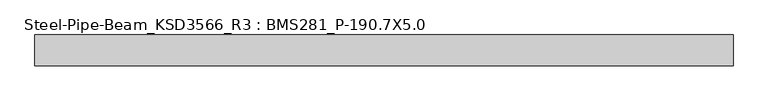
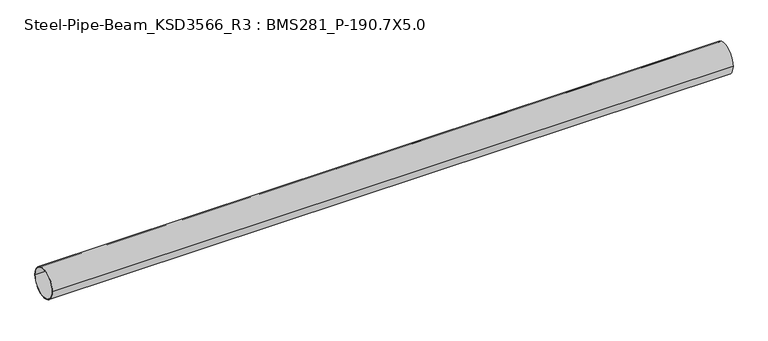
"""IFC4 building model written with IfcOpenShell, lengths in millimetres: member geometry, Steel-Pipe-Beam_KSD3566_R3 : BMS281_P-190.7X5.0."""

from ifc_helpers import new_model, si_unit, point, frame, origin, origin_2d, place, context, project, spatial, circle_curve, trimmed, segment, composite_curve, outline, extrude, source, transform, mapped, element, save


def steel_pipe_beam_ksd3566_r3_bms281_p_190_7x5_0_6dfe9fc3(model_context):
    return source(origin(), model_context, "Body", "SweptSolid", [
        extrude(outline(composite_curve([segment(trimmed(circle_curve(origin_2d(), 95.35), [point((-95.35, 0.0))], [point((95.35, 0.0))], False, "CARTESIAN"), True, "CONTINUOUS"), segment(trimmed(circle_curve(origin_2d(), 95.35), [point((95.35, 0.0))], [point((-95.35, 0.0))], False, "CARTESIAN"), True, "CONTINUOUS")], self_intersect=False), holes=[composite_curve([segment(trimmed(circle_curve(origin_2d(), 90.35), [point((90.35, 0.0))], [point((-90.35, 0.0))], True, "CARTESIAN"), True, "CONTINUOUS"), segment(trimmed(circle_curve(origin_2d(), 90.35), [point((-90.35, 0.0))], [point((90.35, 0.0))], True, "CARTESIAN"), True, "CONTINUOUS")], self_intersect=False)]), frame((-2227.6376817, 0.0, 0.0), z_axis=(1.0, 0.0, 0.0), x_axis=(0.0, 1.0, 0.0)), (0.0, 0.0, 1.0), 4330.1800755),
    ])


if __name__ == "__main__":
    model = new_model("IFC4")
    model_context = context("Model", 3, world=origin())
    ifc_project = project(units=[si_unit("LENGTHUNIT", "METRE", prefix="MILLI")], contexts=[model_context])
    site = spatial("IfcSite", under=ifc_project)
    building = spatial("IfcBuilding", under=site)
    placement = place(None, origin())
    steel_pipe_beam_ksd3566_r3_bms281_p_190_7x5_0_shape = steel_pipe_beam_ksd3566_r3_bms281_p_190_7x5_0_6dfe9fc3(model_context)
    element("IfcMember", 1, ObjectType="Steel-Pipe-Beam_KSD3566_R3 : BMS281_P-190.7X5.0", at=placement, inside=building, context=model_context, shape_type="MappedRepresentation", body=[
        mapped(steel_pipe_beam_ksd3566_r3_bms281_p_190_7x5_0_shape, transform((0.0, 0.0, 0.0), x_axis=(1.0, 0.0, 0.0), y_axis=(0.0, 1.0, 0.0), z_axis=(0.0, 0.0, 1.0))),
    ])
    save(model, "model.ifc")

# Revit data of these elements
# Type "Steel-Pipe-Beam_KSD3566_R3 : BMS281_P-190.7X5.0"
#   Keynote = "P-190.7X5.0"
#   SteelWeight = "Light"
#   t = 0.0050 m
#   Surface Area = 0.599102 m²/m
#   Section Area = 29.1697 cm²
#   Mass per Unit Length = 22.8982 kg/m
#   Length [instance default] = 1.5000 m
#   D = 0.1907 m
#   hec_material4 [instance default] = none
#   hec_material3 [instance default] = none
#   hec_material2 [instance default] = none
#   hec_material1 [instance default] = none
#   Structural Material [instance default] = Steel, 45-345
#   Assembly Code = ""
# Element 1 (IfcMember, "Steel-Pipe-Beam_KSD3566_R3 : BMS281_P-190.7X5.0")
#   Structural Material = none
# Materials
#   "Steel, 45-345": class "Metal", colour RGB 189 187 185, transparency 0, Description = "Steel 345 MPa", Cost = 0
